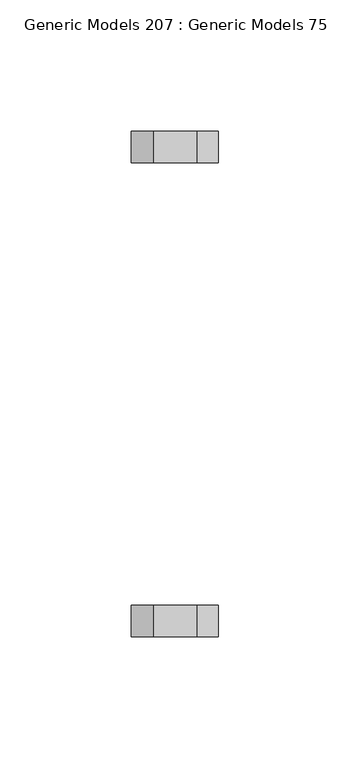
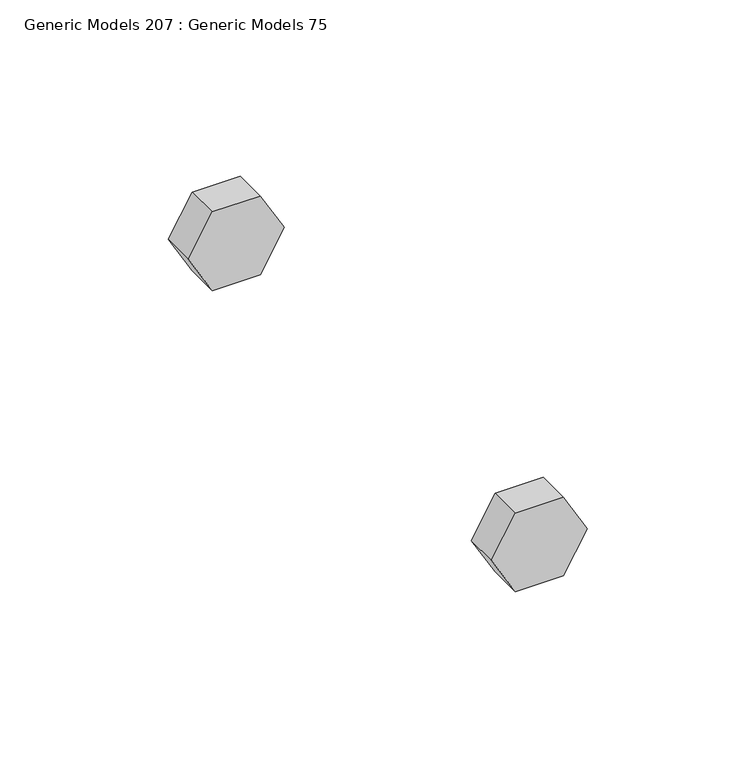
"""IFC4 building model written with IfcOpenShell, lengths in millimetres: proxy geometry, Generic Models 207 : Generic Models 75."""

from ifc_helpers import new_model, si_unit, frame, origin, place, context, project, spatial, polyline, outline, extrude, source, transform, mapped, element, save


def generic_models_207_generic_models_75_89b729dd(model_context):
    return source(origin(), model_context, "Body", "SweptSolid", [
        extrude(outline(polyline([(271657.7625, 31978.2851858), (271657.7625, 31994.7829698), (271672.05, 32003.0318618), (271686.3375, 31994.7829698), (271686.3375, 31978.2851858), (271672.05, 31970.0362939), (271657.7625, 31978.2851858)])), frame((0.0, 30678.2969112, 0.0), z_axis=(0.0, 1.0, 0.0), x_axis=(0.0, 0.0, 1.0)), (0.0, 0.0, 1.0), 11.90625),
        extrude(outline(polyline([(271657.7625, 31978.2851858), (271657.7625, 31994.7829698), (271672.05, 32003.0318618), (271686.3375, 31994.7829698), (271686.3375, 31978.2851858), (271672.05, 31970.0362939), (271657.7625, 31978.2851858)])), frame((0.0, 30858.4781612, 0.0), z_axis=(0.0, 1.0, 0.0), x_axis=(0.0, 0.0, 1.0)), (0.0, 0.0, 1.0), 11.90625),
    ])


if __name__ == "__main__":
    model = new_model("IFC4")
    model_context = context("Model", 3, world=origin())
    ifc_project = project(units=[si_unit("LENGTHUNIT", "METRE", prefix="MILLI")], contexts=[model_context])
    site = spatial("IfcSite", under=ifc_project)
    building = spatial("IfcBuilding", under=site)
    placement = place(None, origin())
    generic_models_207_generic_models_75_shape = generic_models_207_generic_models_75_89b729dd(model_context)
    element("IfcBuildingElementProxy", 1, Name="Generic Models 207 : Generic Models 75", ObjectType="Generic Models 207 : Generic Models 75", at=placement, inside=building, context=model_context, shape_type="MappedRepresentation", body=[
        mapped(generic_models_207_generic_models_75_shape, transform((0.0, 0.0, 0.0), x_axis=(1.0, 0.0, 0.0), y_axis=(0.0, 1.0, 0.0), z_axis=(0.0, 0.0, 1.0))),
    ])
    save(model, "model.ifc")

# Revit data of these elements
# Element 1 (IfcBuildingElementProxy, "Generic Models 207 : Generic Models 75")
#   Materials on its faces: "3/4\" GALV. THRU BOLTS"
# Materials
#   "3/4\" GALV. THRU BOLTS": class "Generic", colour RGB 105 69 171, transparency 0, Cost = 0
